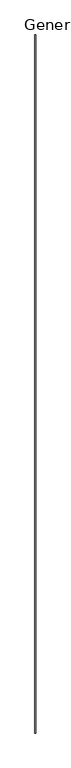
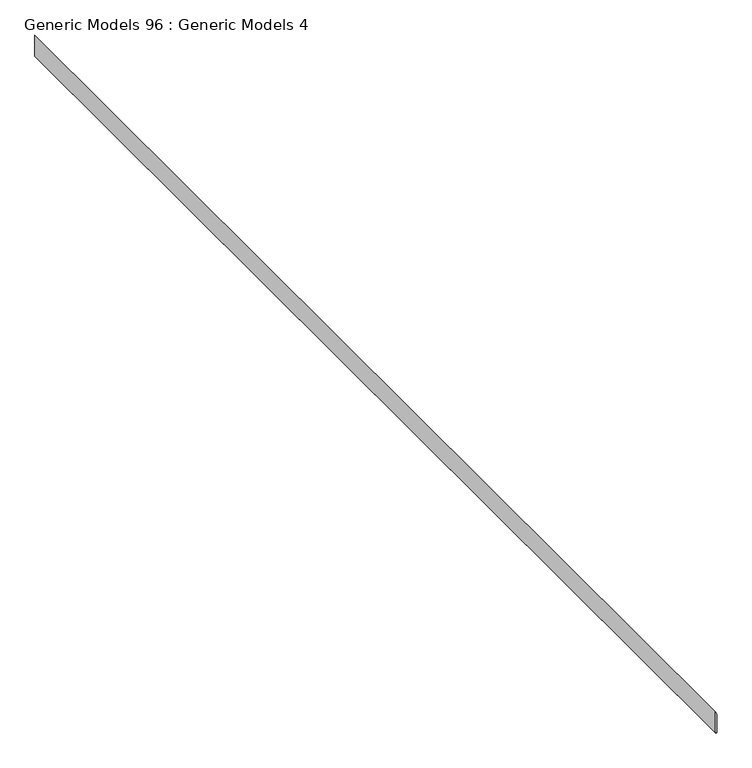
"""IFC4 building model written with IfcOpenShell, lengths in millimetres: proxy geometry, Generic Models 96 : Generic Models 4."""

from ifc_helpers import new_model, si_unit, frame, origin, place, context, project, spatial, polyline, outline, extrude, source, transform, mapped, element, save


def generic_models_96_generic_models_4_fb42b205(model_context):
    return source(origin(), model_context, "Body", "SweptSolid", [
        extrude(outline(polyline([(126689.866, -8877.1781401), (126918.8908545, -8877.1781401), (126953.515065, -8894.9581401), (126693.3458, -8894.9581401), (126693.3458, -8893.6881401), (126689.866, -8893.6881401), (126689.866, -8877.1781401)])), frame((0.0, -6864.9230338, 0.0), z_axis=(0.0, 1.0, 0.0), x_axis=(0.0, 0.0, 1.0)), (0.0, 0.0, 1.0), 13919.2),
    ])


if __name__ == "__main__":
    model = new_model("IFC4")
    model_context = context("Model", 3, world=origin())
    ifc_project = project(units=[si_unit("LENGTHUNIT", "METRE", prefix="MILLI")], contexts=[model_context])
    site = spatial("IfcSite", under=ifc_project)
    building = spatial("IfcBuilding", under=site)
    placement = place(None, origin())
    generic_models_96_generic_models_4_shape = generic_models_96_generic_models_4_fb42b205(model_context)
    element("IfcBuildingElementProxy", 1, Name="Generic Models 96 : Generic Models 4", ObjectType="Generic Models 96 : Generic Models 4", at=placement, inside=building, context=model_context, shape_type="MappedRepresentation", body=[
        mapped(generic_models_96_generic_models_4_shape, transform((0.0, 0.0, 0.0), x_axis=(1.0, 0.0, 0.0), y_axis=(0.0, 1.0, 0.0), z_axis=(0.0, 0.0, 1.0))),
    ])
    save(model, "model.ifc")

# Revit data of these elements
# Element 1 (IfcBuildingElementProxy, "Generic Models 96 : Generic Models 4")
#   Materials on its faces: "_7/8\" SMOOTH TROWEL EXTERIOR STUCCO (COLOR PER OWNER)"
# Materials
#   "_7/8\" SMOOTH TROWEL EXTERIOR STUCCO (COLOR PER OWNER)": class "Generic", colour RGB 233 233 233, transparency 0, Cost = 0
